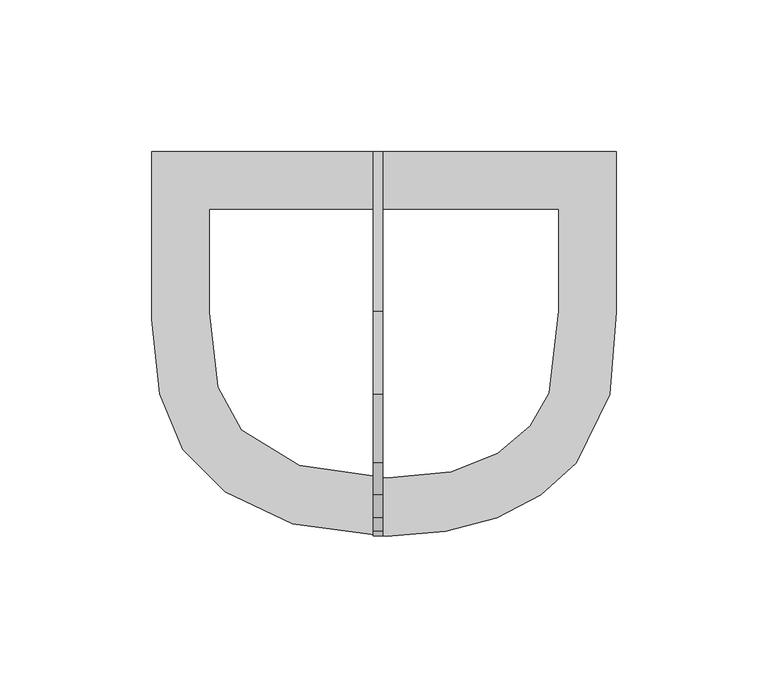
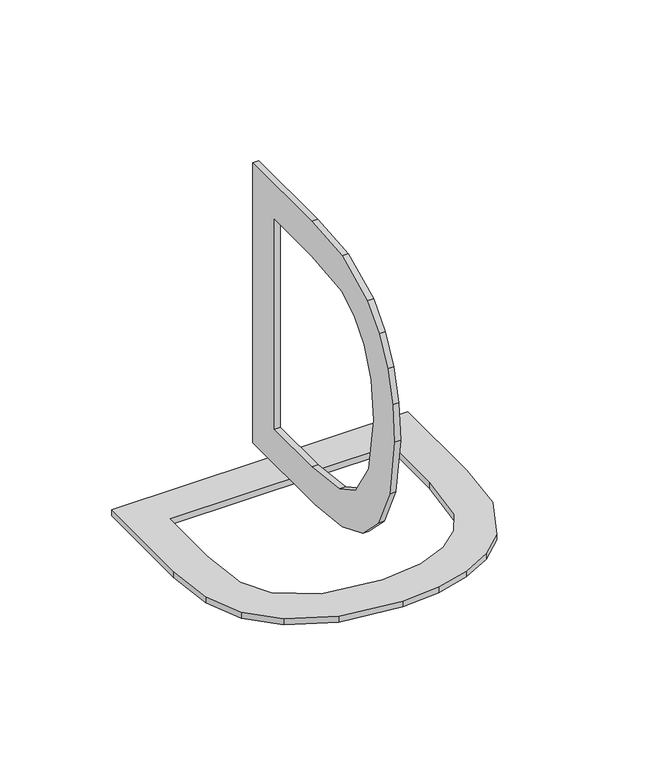
"""IFC4 building model written with IfcOpenShell, lengths in millimetres: proxy geometry, Grid Number2_FedEx : Grid Number2_FedEx."""

from ifc_helpers import new_model, si_unit, frame, origin, origin_with_axes, place, context, project, spatial, polyline, outline, extrude, source, transform, mapped, element, save


def entourage_a6809bf4(model_context):
    return source(origin(), model_context, "Body", "SweptSolid", [
        extrude(outline(polyline([(-184.2739267, 282.3235737), (-31.1785101, 282.3235737), (-31.1785101, 229.5101401), (-33.3837419, 202.1876915), (-44.3351474, 179.6868515), (-55.9967124, 169.0998698), (-70.4989149, 161.5590983), (-87.561429, 157.0458484), (-106.9039286, 155.5414317), (-137.7958626, 159.6155041), (-160.0911302, 170.0810111), (-173.9766154, 184.0599383), (-181.65755, 202.3558871), (-184.2739267, 226.968517), (-184.2739267, 282.3235737)]), holes=[polyline([(-165.1369997, 263.1866466), (-165.1369997, 229.3232561), (-162.3711157, 204.6919378), (-154.5593622, 190.4887497), (-135.553254, 178.8458732), (-106.6049141, 174.6783588), (-85.7486537, 176.7200671), (-70.3494077, 182.845192), (-59.7717703, 191.8950522), (-53.3803356, 202.7109668), (-50.3154372, 229.8465314), (-50.3154372, 263.1866466), (-165.1369997, 263.1866466)])]), origin_with_axes(), (0.0, 0.0, 1.0), 3.175),
        extrude(outline(polyline([(282.3235737, 14.2382753), (226.968517, 14.2382753), (202.3558871, 16.8546521), (184.0599383, 24.5355867), (170.0810111, 38.4210718), (159.6155041, 60.7163394), (155.5414317, 91.6082735), (157.0458484, 110.950773), (161.5590983, 128.0132871), (169.0998698, 142.5154897), (179.6868515, 154.1770546), (202.1876915, 165.1284601), (229.5101401, 167.333692), (282.3235737, 167.333692), (282.3235737, 14.2382753)]), holes=[polyline([(263.1866466, 33.3752024), (263.1866466, 148.1967649), (229.8465314, 148.1967649), (202.7109668, 145.1318664), (191.8950522, 138.7404318), (182.845192, 128.1627943), (176.7200671, 112.7635483), (174.6783588, 91.907288), (178.8458732, 62.9589481), (190.4887497, 43.9528398), (204.6919378, 36.1410864), (229.3232561, 33.3752024), (263.1866466, 33.3752024)])]), frame((-111.2489267, 0.0, 0.0), z_axis=(1.0, 0.0, 0.0), x_axis=(0.0, 1.0, 0.0)), (0.0, 0.0, 1.0), 3.175),
    ])


if __name__ == "__main__":
    model = new_model("IFC4")
    model_context = context("Model", 3, world=origin())
    ifc_project = project(units=[si_unit("LENGTHUNIT", "METRE", prefix="MILLI")], contexts=[model_context])
    site = spatial("IfcSite", under=ifc_project)
    building = spatial("IfcBuilding", under=site)
    placement = place(None, origin())
    entourage_shape = entourage_a6809bf4(model_context)
    element("IfcBuildingElementProxy", 1, Name="Grid Number2_FedEx : Grid Number2_FedEx", ObjectType="Grid Number2_FedEx : Grid Number2_FedEx", at=placement, inside=building, context=model_context, shape_type="MappedRepresentation", body=[
        mapped(entourage_shape, transform((0.0, 0.0, 0.0), x_axis=(1.0, 0.0, 0.0), y_axis=(0.0, 1.0, 0.0), z_axis=(0.0, 0.0, 1.0))),
    ])
    save(model, "model.ifc")

# Revit data of these elements
# Type "Grid Number2_FedEx : Grid Number2_FedEx"
#   Grid [instance default] = "S"
#   Label Width [instance default] = 1' - 0"
#   Half Box Width2 [instance default] = 0' - 6.13846"
#   Half Box Width [instance default] = 0' - 6"
#   Robust [instance default] = yes
#   Height = 0
#   Assembly Code = ""
# Element 1 (IfcBuildingElementProxy, "Grid Number2_FedEx : Grid Number2_FedEx")
#   Grid = "D"
#   Robust = no
#   Materials on its faces: "Letter"
# Materials
#   "Letter": class "Unassigned", colour RGB 178 187 30, transparency 0, Comments = "Rendering appearance not upgraded "
